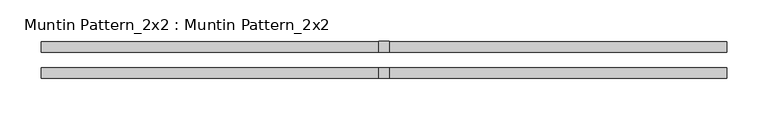
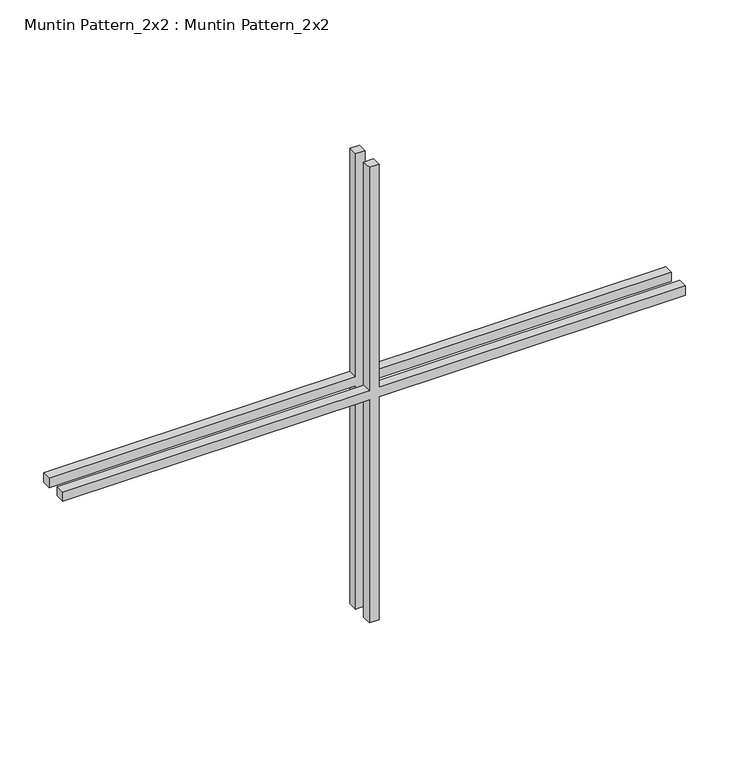
"""IFC4 building model written with IfcOpenShell, lengths in millimetres: proxy geometry, Muntin Pattern_2x2 : Muntin Pattern_2x2."""

import ifcopenshell
import ifcopenshell.guid

model = None  # the IFC model being written
_history = None  # IfcOwnerHistory: only IFC2X3 demands one
_inside = {}  # id of a spatial element -> (the spatial element, [elements in it])
_under = {}  # id of a project, library or spatial element -> (it, [spatial elements below it])
_declared = {}  # id of a project -> (the project, [libraries it declares])
_typed = {}  # id of a type object -> (the type object, [elements of that type])
_made_of = {}  # id of a material, layer set ... -> (it, [elements and type objects made of it])


def new_model(schema):
    """Start an empty IFC model of exactly this schema.

    Asked for "IFC4X3", IfcOpenShell would pick the latest addendum, in which some entities
    have other attributes; the version numbers below select the first issue.
    IFC2X3 requires an IfcOwnerHistory on every rooted entity: one is made here for all.
    """
    global model, _history
    if schema == "IFC4X3":
        model = ifcopenshell.file(schema_version=(4, 3, 0, 0))
    else:
        model = ifcopenshell.file(schema=schema)
    _inside.clear()
    _under.clear()
    _declared.clear()
    _typed.clear()
    _made_of.clear()
    _history = None
    if model.schema == "IFC2X3":
        org = make("IfcOrganization", Name="unknown")
        user = make(
            "IfcPersonAndOrganization",
            ThePerson=make("IfcPerson", FamilyName="unknown"),
            TheOrganization=org,
        )
        app = make(
            "IfcApplication",
            ApplicationDeveloper=org,
            Version="unknown",
            ApplicationFullName="unknown",
            ApplicationIdentifier="unknown",
        )
        _history = make(
            "IfcOwnerHistory",
            OwningUser=user,
            OwningApplication=app,
            ChangeAction="ADDED",
            CreationDate=0,
        )
    return model


def make(cls, **values):
    """One entity of the class cls with the attributes given. An attribute that is None is left unset."""
    return model.create_entity(
        cls, **{name: value for name, value in values.items() if value is not None}
    )


def rooted(cls, **values):
    """An entity with a GlobalId (a new one), such as an element, a storey or a relation."""
    return make(cls, GlobalId=ifcopenshell.guid.new(), OwnerHistory=_history, **values)


def si_unit(unit_type, name, prefix=None):
    """IfcSIUnit, for example si_unit("LENGTHUNIT", "METRE", prefix="MILLI")."""
    return make("IfcSIUnit", UnitType=unit_type, Prefix=prefix, Name=name)


def assignment(units):
    """IfcUnitAssignment: the units of a project."""
    return None if units is None else make("IfcUnitAssignment", Units=units)


def point(xyz):
    """IfcCartesianPoint."""
    return None if xyz is None else make("IfcCartesianPoint", Coordinates=xyz)


def direction(xyz):
    """IfcDirection."""
    return None if xyz is None else make("IfcDirection", DirectionRatios=xyz)


def frame(location, z_axis=None, x_axis=None):
    """IfcAxis2Placement3D, a coordinate frame: its origin and axes. An axis left out is left unset."""
    return make(
        "IfcAxis2Placement3D",
        Location=point(location),
        Axis=direction(z_axis),
        RefDirection=direction(x_axis),
    )


def origin():
    """The frame at (0, 0, 0) with its axes left unset."""
    return frame((0.0, 0.0, 0.0))


def place(relative_to, where):
    """IfcLocalPlacement: puts the frame where relative to a parent placement (None: the world)."""
    return make(
        "IfcLocalPlacement", PlacementRelTo=relative_to, RelativePlacement=where
    )


def context(
    kind, dimensions, precision=None, world=None, true_north=None, identifier=None
):
    """IfcGeometricRepresentationContext, for example the 3D "Model" context."""
    return make(
        "IfcGeometricRepresentationContext",
        ContextIdentifier=identifier,
        ContextType=kind,
        CoordinateSpaceDimension=dimensions,
        Precision=precision,
        WorldCoordinateSystem=world,
        TrueNorth=true_north,
    )


def project(units=None, contexts=None):
    """IfcProject with its units and contexts."""
    return rooted(
        "IfcProject",
        Name="project",
        RepresentationContexts=contexts,
        UnitsInContext=assignment(units),
    )


def spatial(cls, under=None, at=None, **own):
    """A site, building, storey or space (cls), placed at a placement, below another one or the project."""
    s = rooted(cls, ObjectPlacement=at, **own)
    if under is not None:
        _under.setdefault(under.id(), (under, []))[1].append(s)
    return s


def polyline(points):
    """IfcPolyline through the points."""
    return make("IfcPolyline", Points=[point(p) for p in points])


def outline(outer, holes=None, kind="AREA"):
    """IfcArbitraryClosedProfileDef: a profile drawn as a closed curve; with holes, ...WithVoids."""
    if holes is None:
        return make("IfcArbitraryClosedProfileDef", ProfileType=kind, OuterCurve=outer)
    return make(
        "IfcArbitraryProfileDefWithVoids",
        ProfileType=kind,
        OuterCurve=outer,
        InnerCurves=holes,
    )


def extrude(swept, where, along, depth):
    """IfcExtrudedAreaSolid: the profile swept, set in the frame where, extruded along a direction by depth."""
    return make(
        "IfcExtrudedAreaSolid",
        SweptArea=swept,
        Position=where,
        ExtrudedDirection=direction(along),
        Depth=depth,
    )


def shape(context_of_items, identifier, shape_type, items):
    """IfcShapeRepresentation: the items that make up one representation, for example the "Body"."""
    return make(
        "IfcShapeRepresentation",
        ContextOfItems=context_of_items,
        RepresentationIdentifier=identifier,
        RepresentationType=shape_type,
        Items=items,
    )


def source(mapping_origin, context_of_items, identifier, shape_type, items):
    """IfcRepresentationMap: a shape defined once, which mapped items show again and again."""
    return make(
        "IfcRepresentationMap",
        MappingOrigin=mapping_origin,
        MappedRepresentation=shape(context_of_items, identifier, shape_type, items),
    )


def transform(
    local_origin,
    x_axis=None,
    y_axis=None,
    z_axis=None,
    scale=None,
    scale2=None,
    scale3=None,
    uniform=True,
):
    """IfcCartesianTransformationOperator3D, or its non-uniform kind. x_axis, y_axis, z_axis: its Axis1, 2, 3."""
    if uniform:
        return make(
            "IfcCartesianTransformationOperator3D",
            Axis1=direction(x_axis),
            Axis2=direction(y_axis),
            LocalOrigin=point(local_origin),
            Scale=scale,
            Axis3=direction(z_axis),
        )
    return make(
        "IfcCartesianTransformationOperator3DnonUniform",
        Axis1=direction(x_axis),
        Axis2=direction(y_axis),
        LocalOrigin=point(local_origin),
        Scale=scale,
        Axis3=direction(z_axis),
        Scale2=scale2,
        Scale3=scale3,
    )


def mapped(mapping_source, mapping_target):
    """IfcMappedItem: shows the shape of a source again, moved by a transform."""
    return make(
        "IfcMappedItem", MappingSource=mapping_source, MappingTarget=mapping_target
    )


def made_of(thing, what):
    """Note that an element or type object is made of a material, layer set ...; save() writes the relation."""
    if what is not None:
        _made_of.setdefault(what.id(), (what, []))[1].append(thing)
    return thing


def element(
    cls,
    number,
    at=None,
    inside=None,
    cuts=None,
    type_object=None,
    material=None,
    context=None,
    identifier="Body",
    shape_type=None,
    held_by="IfcProductDefinitionShape",
    body=None,
    shapes=None,
    **own,
):
    """One element of the class cls, such as IfcWall. Its Tag is "e" and its number.

    at: its placement. inside: the storey or other place that contains it. cuts: it is an
    opening in that element (IfcRelVoidsElement). A single representation is given by context,
    identifier, shape_type and body (its items); several are given by shapes. held_by: the class
    of the entity that holds the representations. save() writes the other relations.
    """
    e = rooted(cls, Tag="e%d" % number, ObjectPlacement=at, **own)
    if body is not None:
        shapes = [shape(context, identifier, shape_type, body)]
    if shapes is not None:
        e.Representation = make(held_by, Representations=shapes)
    if inside is not None:
        _inside.setdefault(inside.id(), (inside, []))[1].append(e)
    if cuts is not None:
        rooted(
            "IfcRelVoidsElement", RelatingBuildingElement=cuts, RelatedOpeningElement=e
        )
    if type_object is not None:
        _typed.setdefault(type_object.id(), (type_object, []))[1].append(e)
    return made_of(e, material)


def aggregate(whole, parts):
    """IfcRelAggregates: a whole, such as a stair, and the parts it consists of."""
    return rooted("IfcRelAggregates", RelatingObject=whole, RelatedObjects=parts)


def save(model, path):
    """Write the relations noted so far, then the file.

    IfcRelAggregates (storeys below a building ...), IfcRelContainedInSpatialStructure (elements
    in a storey), IfcRelDefinesByType, IfcRelAssociatesMaterial and IfcRelDeclares: one each for
    every whole, place, type object, material and project.
    """
    for whole, parts in _under.values():
        aggregate(whole, parts)
    for where, things in _inside.values():
        rooted(
            "IfcRelContainedInSpatialStructure",
            RelatedElements=things,
            RelatingStructure=where,
        )
    for kind, things in _typed.values():
        rooted("IfcRelDefinesByType", RelatedObjects=things, RelatingType=kind)
    for what, things in _made_of.values():
        rooted("IfcRelAssociatesMaterial", RelatedObjects=things, RelatingMaterial=what)
    for by, libraries in _declared.values():
        rooted("IfcRelDeclares", RelatingContext=by, RelatedDefinitions=libraries)
    model.write(path)


def muntin_pattern_2x2_muntin_pattern_2x2_9cade0ad(model_context):
    return source(origin(), model_context, "Body", "SweptSolid", [
        extrude(outline(polyline([(325.4375, -6.35), (325.4375, -412.75), (312.7375, -412.75), (312.7375, -6.35), (0.0, -6.35), (0.0, 6.35), (312.7375, 6.35), (312.7375, 412.75), (325.4375, 412.75), (325.4375, 6.35), (638.175, 6.35), (638.175, -6.35), (325.4375, -6.35)])), frame((0.0, -22.225, 0.0), z_axis=(0.0, 1.0, 0.0), x_axis=(0.0, 0.0, 1.0)), (0.0, 0.0, 1.0), 12.7),
        extrude(outline(polyline([(325.4375, -6.35), (325.4375, -412.75), (312.7375, -412.75), (312.7375, -6.35), (0.0, -6.35), (0.0, 6.35), (312.7375, 6.35), (312.7375, 412.75), (325.4375, 412.75), (325.4375, 6.35), (638.175, 6.35), (638.175, -6.35), (325.4375, -6.35)])), frame((0.0, 9.525, 0.0), z_axis=(0.0, 1.0, 0.0), x_axis=(0.0, 0.0, 1.0)), (0.0, 0.0, 1.0), 12.7),
    ])


if __name__ == "__main__":
    model = new_model("IFC4")
    model_context = context("Model", 3, world=origin())
    ifc_project = project(units=[si_unit("LENGTHUNIT", "METRE", prefix="MILLI")], contexts=[model_context])
    site = spatial("IfcSite", under=ifc_project)
    building = spatial("IfcBuilding", under=site)
    placement = place(None, origin())
    muntin_pattern_2x2_muntin_pattern_2x2_shape = muntin_pattern_2x2_muntin_pattern_2x2_9cade0ad(model_context)
    element("IfcBuildingElementProxy", 1, Name="Muntin Pattern_2x2 : Muntin Pattern_2x2", ObjectType="Muntin Pattern_2x2 : Muntin Pattern_2x2", at=placement, inside=building, context=model_context, shape_type="MappedRepresentation", body=[
        mapped(muntin_pattern_2x2_muntin_pattern_2x2_shape, transform((0.0, 0.0, 0.0), x_axis=(1.0, 0.0, 0.0), y_axis=(0.0, 1.0, 0.0), z_axis=(0.0, 0.0, 1.0))),
    ])
    save(model, "model.ifc")

# Revit data of these elements
# Type "Muntin Pattern_2x2 : Muntin Pattern_2x2"
#   Width [instance default] = 4' - 0"
#   Thickness = 0' - 0 1/2"
#   Height [instance default] = 4' - 0"
#   Distance = 0' - 0 3/4"
#   Interior Material [instance default] = none
#   Exterior Material [instance default] = none
# Element 1 (IfcBuildingElementProxy, "Muntin Pattern_2x2 : Muntin Pattern_2x2")
#   Width = 2' - 8 1/2"
#   Height = 2' - 1 1/8"
#   Interior Material = Wood - Stained
#   Exterior Material = Clad - White
#   Materials on its faces: "Clad - White", "Wood - Stained"
# Materials
#   "Clad - White": class "Wood", colour RGB 242 242 238, transparency 0, Cost = 0
#   "Wood - Stained": class "Wood", colour RGB 224 178 126, transparency 0, Cost = 0
